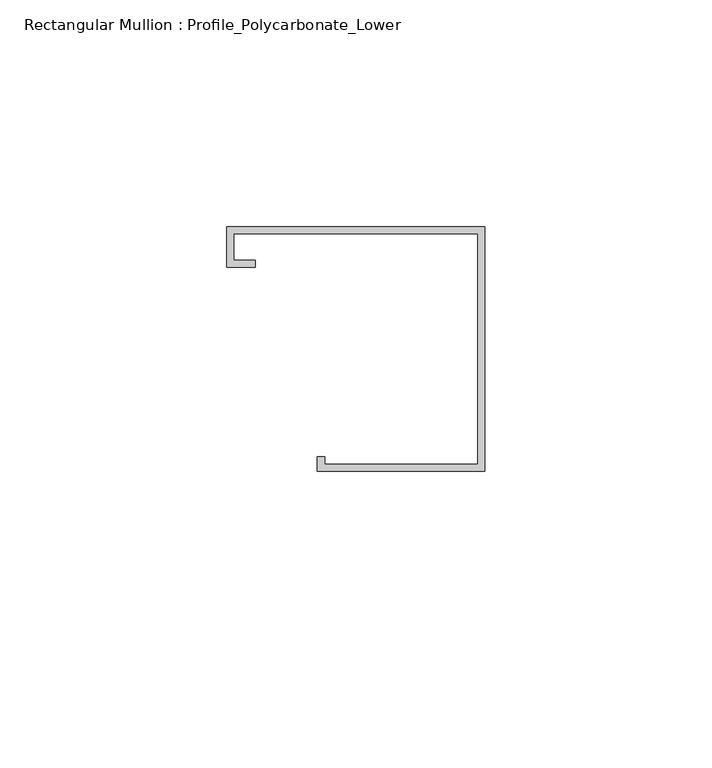
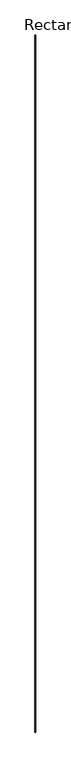
"""IFC4 building model written with IfcOpenShell, lengths in millimetres: member geometry, Rectangular Mullion : Profile_Polycarbonate_Lower."""

from ifc_helpers import new_model, si_unit, frame, origin, place, context, project, spatial, polyline, outline, extrude, source, transform, mapped, element, save


def rectangular_mullion_profile_polycarbonate_lower_b4fa1ed4(model_context):
    return source(origin(), model_context, "Body", "SweptSolid", [
        extrude(outline(polyline([(0.0, 28.984575), (0.0, -25.015825), (-36.9824, -25.015825), (-36.9824, -21.840825), (-35.3949, -21.840825), (-35.3949, -23.428325), (-1.5875, -23.428325), (-1.5875, 27.397075), (-55.4101, 27.397075), (-55.4101, 21.580475), (-50.6476, 21.580475), (-50.6476, 19.992975), (-56.9976, 19.992975), (-56.9976, 28.984575), (0.0, 28.984575)])), frame((0.0, 0.0, -88557.2778), z_axis=(0.0, 0.0, 1.0), x_axis=(1.0, 0.0, 0.0)), (0.0, 0.0, 1.0), 88557.2778),
    ])


if __name__ == "__main__":
    model = new_model("IFC4")
    model_context = context("Model", 3, world=origin())
    ifc_project = project(units=[si_unit("LENGTHUNIT", "METRE", prefix="MILLI")], contexts=[model_context])
    site = spatial("IfcSite", under=ifc_project)
    building = spatial("IfcBuilding", under=site)
    placement = place(None, origin())
    rectangular_mullion_profile_polycarbonate_lower_shape = rectangular_mullion_profile_polycarbonate_lower_b4fa1ed4(model_context)
    element("IfcMember", 1, ObjectType="Rectangular Mullion : Profile_Polycarbonate_Lower", at=placement, inside=building, context=model_context, shape_type="MappedRepresentation", body=[
        mapped(rectangular_mullion_profile_polycarbonate_lower_shape, transform((0.0, 0.0, 0.0), x_axis=(1.0, 0.0, 0.0), y_axis=(0.0, 1.0, 0.0), z_axis=(0.0, 0.0, 1.0))),
    ])
    save(model, "model.ifc")

# Revit data of these elements
# Type "Rectangular Mullion : Profile_Polycarbonate_Lower"
#   built-in parameter 1007322 = 0.177167 (stored number, unit not read)
#   built-in parameter 1007321 = 0 (stored number, unit not read)
#   built-in parameter 1007320 = 0.00520833 (stored number, unit not read)
